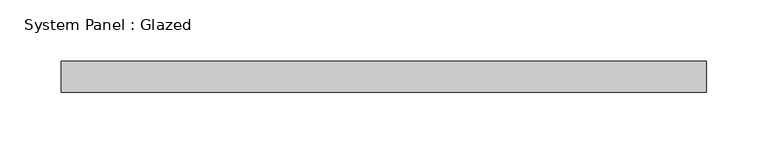
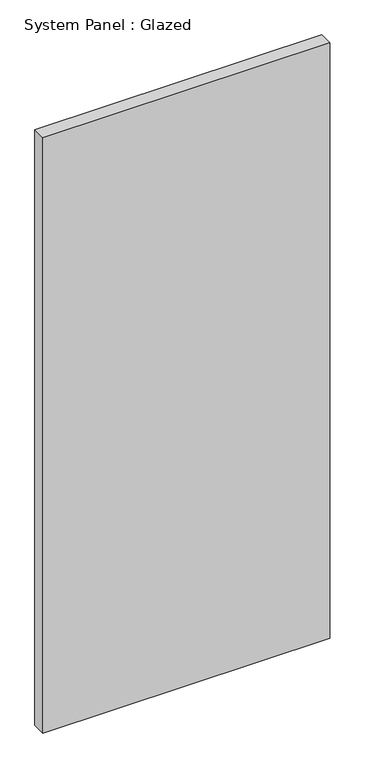
"""IFC4 building model written with IfcOpenShell, lengths in millimetres: plate geometry, System Panel : Glazed."""

from ifc_helpers import new_model, si_unit, origin, origin_with_axes, place, context, project, spatial, polyline, outline, extrude, source, transform, mapped, element, save


def system_panel_glazed_9dcaf0c5(model_context):
    return source(origin(), model_context, "Body", "SweptSolid", [
        extrude(outline(polyline([(263.525, -44.45), (-263.525, -44.45), (-263.525, -19.05), (263.525, -19.05), (263.525, -44.45)])), origin_with_axes(), (0.0, 0.0, 1.0), 1155.7),
    ])


if __name__ == "__main__":
    model = new_model("IFC4")
    model_context = context("Model", 3, world=origin())
    ifc_project = project(units=[si_unit("LENGTHUNIT", "METRE", prefix="MILLI")], contexts=[model_context])
    site = spatial("IfcSite", under=ifc_project)
    building = spatial("IfcBuilding", under=site)
    placement = place(None, origin())
    system_panel_glazed_shape = system_panel_glazed_9dcaf0c5(model_context)
    element("IfcPlate", 1, ObjectType="System Panel : Glazed", at=placement, inside=building, context=model_context, shape_type="MappedRepresentation", body=[
        mapped(system_panel_glazed_shape, transform((0.0, 0.0, 0.0), x_axis=(1.0, 0.0, 0.0), y_axis=(0.0, 1.0, 0.0), z_axis=(0.0, 0.0, 1.0))),
    ])
    save(model, "model.ifc")

# Revit data of these elements
# Element 1 (IfcPlate, "System Panel : Glazed")
#   Materials on its faces: "Glass"
# Materials
#   "Glass": class "Glass", colour RGB 0 128 192, transparency 0.75
